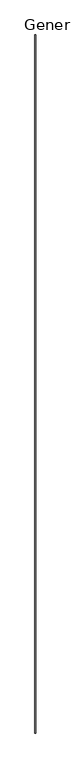
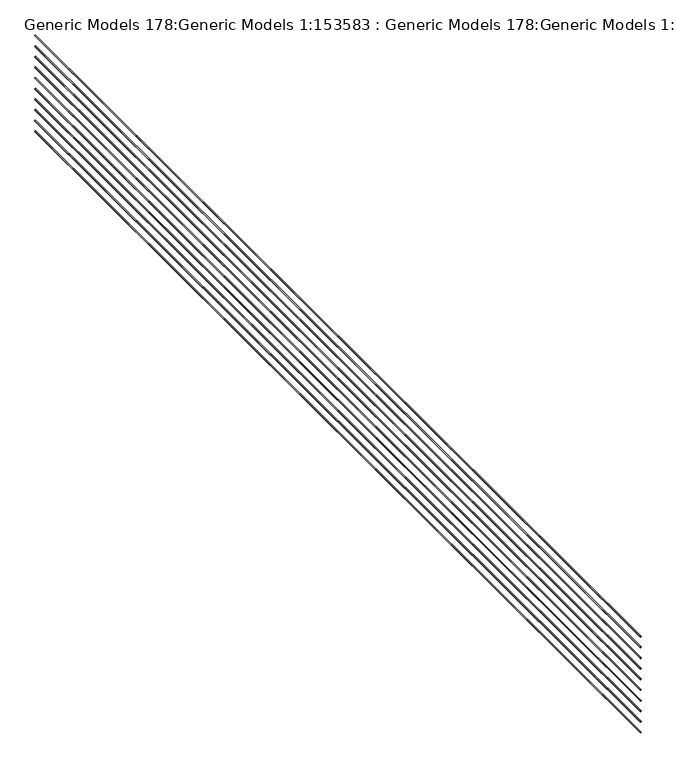
"""IFC4 building model written with IfcOpenShell, lengths in millimetres: proxy geometry, Generic Models 178:Generic Models 1:153583 : Generic Models 178:Generic Models 1:153583."""

from ifc_helpers import new_model, si_unit, point, frame, frame_2d, origin, place, context, project, spatial, circle_curve, trimmed, segment, composite_curve, outline, extrude, source, transform, mapped, element, save


def generic_models_178_generic_models_1_153583_generic_models_7d77c399(model_context):
    return source(origin(), model_context, "Body", "SweptSolid", [
        extrude(outline(composite_curve([segment(trimmed(circle_curve(frame_2d((-165.8350126, -10380.5203813)), 4.7625), [point((-165.8350126, -10385.2828813))], [point((-165.8350126, -10375.7578813))], False, "CARTESIAN"), True, "CONTINUOUS"), segment(trimmed(circle_curve(frame_2d((-165.8350126, -10380.5203813)), 4.7625), [point((-165.8350126, -10375.7578813))], [point((-165.8350126, -10385.2828813))], False, "CARTESIAN"), True, "CONTINUOUS")], self_intersect=False)), frame((0.0, -464.4974793, 0.0), z_axis=(0.0, 1.0, 0.0), x_axis=(0.0, 0.0, 1.0)), (0.0, 0.0, 1.0), 9475.7774227),
        extrude(outline(composite_curve([segment(trimmed(circle_curve(frame_2d((-64.2350126, -10380.5203813)), 4.7625), [point((-64.2350126, -10385.2828813))], [point((-64.2350126, -10375.7578813))], False, "CARTESIAN"), True, "CONTINUOUS"), segment(trimmed(circle_curve(frame_2d((-64.2350126, -10380.5203813)), 4.7625), [point((-64.2350126, -10375.7578813))], [point((-64.2350126, -10385.2828813))], False, "CARTESIAN"), True, "CONTINUOUS")], self_intersect=False)), frame((0.0, -464.4974793, 0.0), z_axis=(0.0, 1.0, 0.0), x_axis=(0.0, 0.0, 1.0)), (0.0, 0.0, 1.0), 9475.7774227),
        extrude(outline(composite_curve([segment(trimmed(circle_curve(frame_2d((37.3649874, -10380.5203813)), 4.7625), [point((37.3649874, -10385.2828813))], [point((37.3649874, -10375.7578813))], False, "CARTESIAN"), True, "CONTINUOUS"), segment(trimmed(circle_curve(frame_2d((37.3649874, -10380.5203813)), 4.7625), [point((37.3649874, -10375.7578813))], [point((37.3649874, -10385.2828813))], False, "CARTESIAN"), True, "CONTINUOUS")], self_intersect=False)), frame((0.0, -464.4974793, 0.0), z_axis=(0.0, 1.0, 0.0), x_axis=(0.0, 0.0, 1.0)), (0.0, 0.0, 1.0), 9475.7774227),
        extrude(outline(composite_curve([segment(trimmed(circle_curve(frame_2d((138.9649874, -10380.5203813)), 4.7625), [point((138.9649874, -10385.2828813))], [point((138.9649874, -10375.7578813))], False, "CARTESIAN"), True, "CONTINUOUS"), segment(trimmed(circle_curve(frame_2d((138.9649874, -10380.5203813)), 4.7625), [point((138.9649874, -10375.7578813))], [point((138.9649874, -10385.2828813))], False, "CARTESIAN"), True, "CONTINUOUS")], self_intersect=False)), frame((0.0, -464.4974793, 0.0), z_axis=(0.0, 1.0, 0.0), x_axis=(0.0, 0.0, 1.0)), (0.0, 0.0, 1.0), 9475.7774227),
        extrude(outline(composite_curve([segment(trimmed(circle_curve(frame_2d((240.5649874, -10380.5203813)), 4.7625), [point((240.5649874, -10385.2828813))], [point((240.5649874, -10375.7578813))], False, "CARTESIAN"), True, "CONTINUOUS"), segment(trimmed(circle_curve(frame_2d((240.5649874, -10380.5203813)), 4.7625), [point((240.5649874, -10375.7578813))], [point((240.5649874, -10385.2828813))], False, "CARTESIAN"), True, "CONTINUOUS")], self_intersect=False)), frame((0.0, -464.4974793, 0.0), z_axis=(0.0, 1.0, 0.0), x_axis=(0.0, 0.0, 1.0)), (0.0, 0.0, 1.0), 9475.7774227),
        extrude(outline(composite_curve([segment(trimmed(circle_curve(frame_2d((342.1649874, -10380.5203813)), 4.7625), [point((342.1649874, -10385.2828813))], [point((342.1649874, -10375.7578813))], False, "CARTESIAN"), True, "CONTINUOUS"), segment(trimmed(circle_curve(frame_2d((342.1649874, -10380.5203813)), 4.7625), [point((342.1649874, -10375.7578813))], [point((342.1649874, -10385.2828813))], False, "CARTESIAN"), True, "CONTINUOUS")], self_intersect=False)), frame((0.0, -464.4974793, 0.0), z_axis=(0.0, 1.0, 0.0), x_axis=(0.0, 0.0, 1.0)), (0.0, 0.0, 1.0), 9475.7774227),
        extrude(outline(composite_curve([segment(trimmed(circle_curve(frame_2d((443.7649874, -10380.5203813)), 4.7625), [point((443.7649874, -10385.2828813))], [point((443.7649874, -10375.7578813))], False, "CARTESIAN"), True, "CONTINUOUS"), segment(trimmed(circle_curve(frame_2d((443.7649874, -10380.5203813)), 4.7625), [point((443.7649874, -10375.7578813))], [point((443.7649874, -10385.2828813))], False, "CARTESIAN"), True, "CONTINUOUS")], self_intersect=False)), frame((0.0, -464.4974793, 0.0), z_axis=(0.0, 1.0, 0.0), x_axis=(0.0, 0.0, 1.0)), (0.0, 0.0, 1.0), 9475.7774227),
        extrude(outline(composite_curve([segment(trimmed(circle_curve(frame_2d((545.3649874, -10380.5203813)), 4.7625), [point((545.3649874, -10385.2828813))], [point((545.3649874, -10375.7578813))], False, "CARTESIAN"), True, "CONTINUOUS"), segment(trimmed(circle_curve(frame_2d((545.3649874, -10380.5203813)), 4.7625), [point((545.3649874, -10375.7578813))], [point((545.3649874, -10385.2828813))], False, "CARTESIAN"), True, "CONTINUOUS")], self_intersect=False)), frame((0.0, -464.4974793, 0.0), z_axis=(0.0, 1.0, 0.0), x_axis=(0.0, 0.0, 1.0)), (0.0, 0.0, 1.0), 9475.7774227),
        extrude(outline(composite_curve([segment(trimmed(circle_curve(frame_2d((646.9649874, -10380.5203813)), 4.7625), [point((646.9649874, -10385.2828813))], [point((646.9649874, -10375.7578813))], False, "CARTESIAN"), True, "CONTINUOUS"), segment(trimmed(circle_curve(frame_2d((646.9649874, -10380.5203813)), 4.7625), [point((646.9649874, -10375.7578813))], [point((646.9649874, -10385.2828813))], False, "CARTESIAN"), True, "CONTINUOUS")], self_intersect=False)), frame((0.0, -464.4974793, 0.0), z_axis=(0.0, 1.0, 0.0), x_axis=(0.0, 0.0, 1.0)), (0.0, 0.0, 1.0), 9475.7774227),
        extrude(outline(composite_curve([segment(trimmed(circle_curve(frame_2d((748.5649874, -10380.5203813)), 4.7625), [point((748.5649874, -10385.2828813))], [point((748.5649874, -10375.7578813))], False, "CARTESIAN"), True, "CONTINUOUS"), segment(trimmed(circle_curve(frame_2d((748.5649874, -10380.5203813)), 4.7625), [point((748.5649874, -10375.7578813))], [point((748.5649874, -10385.2828813))], False, "CARTESIAN"), True, "CONTINUOUS")], self_intersect=False)), frame((0.0, -464.4974793, 0.0), z_axis=(0.0, 1.0, 0.0), x_axis=(0.0, 0.0, 1.0)), (0.0, 0.0, 1.0), 9475.7774227),
    ])


if __name__ == "__main__":
    model = new_model("IFC4")
    model_context = context("Model", 3, world=origin())
    ifc_project = project(units=[si_unit("LENGTHUNIT", "METRE", prefix="MILLI")], contexts=[model_context])
    site = spatial("IfcSite", under=ifc_project)
    building = spatial("IfcBuilding", under=site)
    placement = place(None, origin())
    generic_models_178_generic_models_1_153583_generic_models_shape = generic_models_178_generic_models_1_153583_generic_models_7d77c399(model_context)
    element("IfcBuildingElementProxy", 1, Name="Generic Models 178:Generic Models 1:153583 : Generic Models 178:Generic Models 1:153583", ObjectType="Generic Models 178:Generic Models 1:153583 : Generic Models 178:Generic Models 1:153583", at=placement, inside=building, context=model_context, shape_type="MappedRepresentation", body=[
        mapped(generic_models_178_generic_models_1_153583_generic_models_shape, transform((0.0, 0.0, 0.0), x_axis=(1.0, 0.0, 0.0), y_axis=(0.0, 1.0, 0.0), z_axis=(0.0, 0.0, 1.0))),
    ])
    save(model, "model.ifc")

# Revit data of these elements
# Type "Generic Models 178:Generic Models 1:153583 : Generic Models 178:Generic Models 1:153583"
#   NameOverride = "Generic Models 178:Generic Models 1:153583"
#   ObjectTypeOverride = "Generic Models 178:Generic Models 1"
#   Reference = "Generic Models 1"
#   Category = "Generic Models"
#   Tag = "153583"
# Element 1 (IfcBuildingElementProxy, "Generic Models 178:Generic Models 1:153583 : Generic Models 178:Generic Models 1:153583")
#   Materials on its faces: "_1/2\" DIA. SOLID STOCK STEEL HORIZONTAL RAILINGS"
# Materials
#   "_1/2\" DIA. SOLID STOCK STEEL HORIZONTAL RAILINGS": class "Metal", colour RGB 199 199 199, transparency 0, Description = "Structural steel 50ksi", Cost = 0
